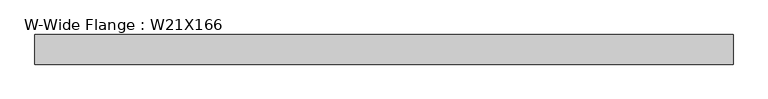
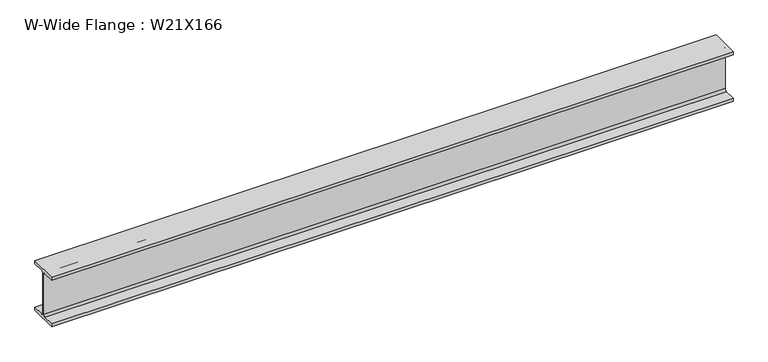
"""IFC4 building model written with IfcOpenShell, lengths in millimetres: beam geometry, W-Wide Flange : W21X166."""

from ifc_helpers import new_model, si_unit, point, frame, frame_2d, origin, place, context, project, spatial, polyline, circle_curve, trimmed, segment, composite_curve, outline, extrude, source, transform, mapped, element, save


def w_wide_flange_w21x166_9585b54c(model_context):
    return source(origin(), model_context, "Body", "SweptSolid", [
        extrude(outline(composite_curve([segment(polyline([(157.48, -251.206), (157.48, -285.75), (-157.48, -285.75), (-157.48, -251.206), (-32.131, -251.206)]), True, "CONTINUOUS"), segment(trimmed(circle_curve(frame_2d((-32.131, -228.6)), 22.606), [point((-32.131, -251.206))], [point((-9.525, -228.6))], True, "CARTESIAN"), True, "CONTINUOUS"), segment(polyline([(-9.525, -228.6), (-9.525, 228.6)]), True, "CONTINUOUS"), segment(trimmed(circle_curve(frame_2d((-32.131, 228.6)), 22.606), [point((-9.525, 228.6))], [point((-32.131, 251.206))], True, "CARTESIAN"), True, "CONTINUOUS"), segment(polyline([(-32.131, 251.206), (-157.48, 251.206), (-157.48, 285.75), (157.48, 285.75), (157.48, 251.206), (32.131, 251.206)]), True, "CONTINUOUS"), segment(trimmed(circle_curve(frame_2d((32.131, 228.6)), 22.606), [point((32.131, 251.206))], [point((9.525, 228.6))], True, "CARTESIAN"), True, "CONTINUOUS"), segment(polyline([(9.525, 228.6), (9.525, -228.6)]), True, "CONTINUOUS"), segment(trimmed(circle_curve(frame_2d((32.131, -228.6)), 22.606), [point((9.525, -228.6))], [point((32.131, -251.206))], True, "CARTESIAN"), True, "CONTINUOUS"), segment(polyline([(32.131, -251.206), (157.48, -251.206)]), True, "CONTINUOUS")], self_intersect=False)), frame((-3708.0520383, 0.0, 0.0), z_axis=(1.0, 0.0, 0.0), x_axis=(0.0, 1.0, 0.0)), (0.0, 0.0, 1.0), 7416.1040767),
    ])


if __name__ == "__main__":
    model = new_model("IFC4")
    model_context = context("Model", 3, world=origin())
    ifc_project = project(units=[si_unit("LENGTHUNIT", "METRE", prefix="MILLI")], contexts=[model_context])
    site = spatial("IfcSite", under=ifc_project)
    building = spatial("IfcBuilding", under=site)
    placement = place(None, origin())
    w_wide_flange_w21x166_shape = w_wide_flange_w21x166_9585b54c(model_context)
    element("IfcBeam", 1, ObjectType="W-Wide Flange : W21X166", at=placement, inside=building, context=model_context, shape_type="MappedRepresentation", body=[
        mapped(w_wide_flange_w21x166_shape, transform((0.0, 0.0, 0.0), x_axis=(1.0, 0.0, 0.0), y_axis=(0.0, 1.0, 0.0), z_axis=(0.0, 0.0, 1.0))),
    ])
    save(model, "model.ifc")

# Revit data of these elements
# Type "W-Wide Flange : W21X166"
#   Assembly Code = "B10"
#   W = 166
#   Length [instance default] = 5' - 0"
#   bf = 1' - 0.4"
#   d = 1' - 10 1/2"
#   k = 0' - 2 1/4"
#   k2 = 0' - 0.89"
#   tf = 0' - 1.36"
#   tw = 0' - 0 3/4"
#   A = 0.338889 SF
#   Structural Material [instance default] = Steel ASTM A992
# Element 1 (IfcBeam, "W-Wide Flange : W21X166")
#   Structural Material = Steel
#   Materials on its faces: "Steel"
# Materials
#   "Steel ASTM A992": class "Metal", colour RGB 199 199 199, transparency 0, Description = "Structural steel 50ksi", Cost = 0
#   "Steel": class "Metal", colour RGB 118 118 114, transparency 0, Description = "Steel, mill finish", Cost = 0
